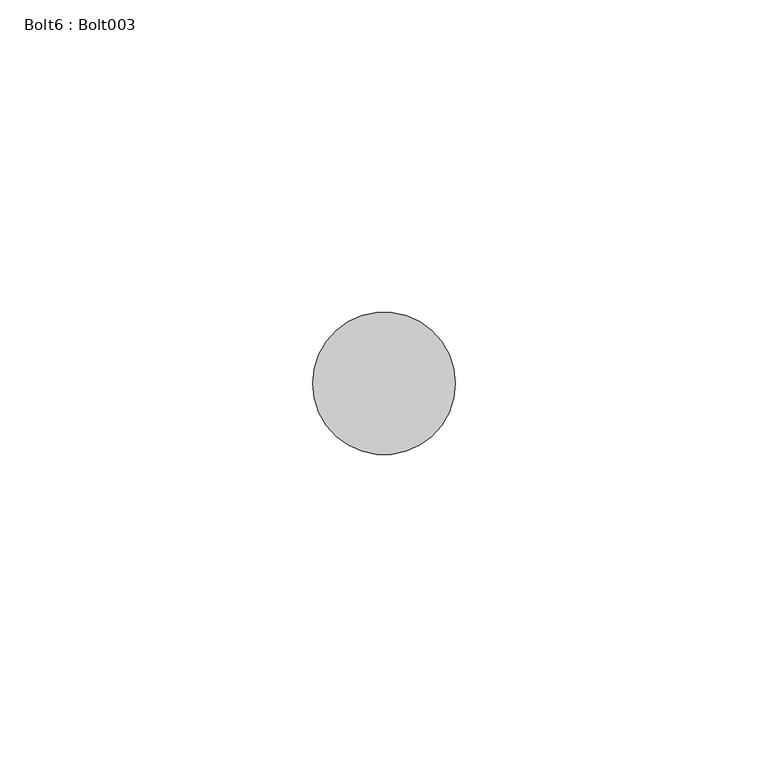
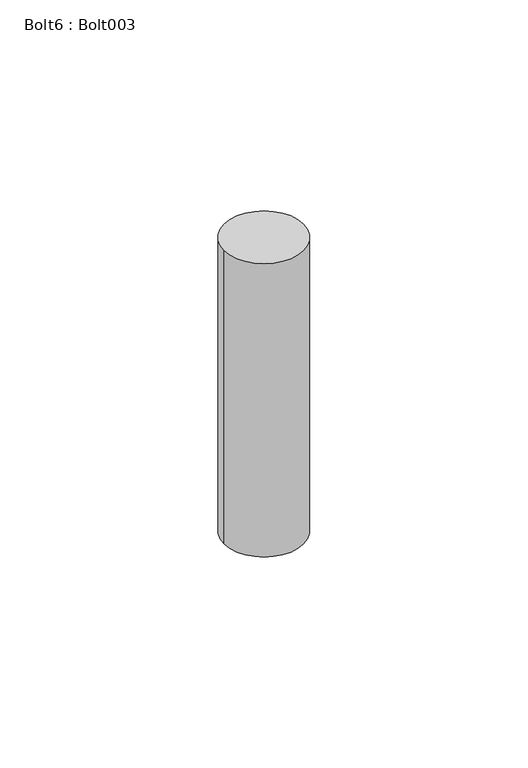
"""IFC4 building model written with IfcOpenShell, lengths in millimetres: proxy geometry, Bolt6 : Bolt003."""

from ifc_helpers import new_model, si_unit, point, frame, frame_2d, origin, place, context, project, spatial, circle_curve, trimmed, segment, composite_curve, outline, extrude, source, transform, mapped, element, save


def bolt6_bolt003_a672977d(model_context):
    return source(origin(), model_context, "Body", "SweptSolid", [
        extrude(outline(composite_curve([segment(trimmed(circle_curve(frame_2d((5172.3828124, 1896.5882072)), 11.4045168), [point((5160.9782956, 1896.5882072))], [point((5183.7873292, 1896.5882072))], False, "CARTESIAN"), True, "CONTINUOUS"), segment(trimmed(circle_curve(frame_2d((5172.3828124, 1896.5882072)), 11.4045168), [point((5183.7873292, 1896.5882072))], [point((5160.9782956, 1896.5882072))], False, "CARTESIAN"), True, "CONTINUOUS")], self_intersect=False)), frame((0.0, 0.0, 36645.5959962), z_axis=(0.0, 0.0, 1.0), x_axis=(1.0, 0.0, 0.0)), (0.0, 0.0, 1.0), 88.9),
    ])


if __name__ == "__main__":
    model = new_model("IFC4")
    model_context = context("Model", 3, world=origin())
    ifc_project = project(units=[si_unit("LENGTHUNIT", "METRE", prefix="MILLI")], contexts=[model_context])
    site = spatial("IfcSite", under=ifc_project)
    building = spatial("IfcBuilding", under=site)
    placement = place(None, origin())
    bolt6_bolt003_shape = bolt6_bolt003_a672977d(model_context)
    element("IfcBuildingElementProxy", 1, Name="Bolt6 : Bolt003", ObjectType="Bolt6 : Bolt003", at=placement, inside=building, context=model_context, shape_type="MappedRepresentation", body=[
        mapped(bolt6_bolt003_shape, transform((0.0, 0.0, 0.0), x_axis=(1.0, 0.0, 0.0), y_axis=(0.0, 1.0, 0.0), z_axis=(0.0, 0.0, 1.0))),
    ])
    save(model, "model.ifc")

# Revit data of these elements
# Type "Bolt6 : Bolt003"
#   NameOverride = "Bolt003"
# Element 1 (IfcBuildingElementProxy, "Bolt6 : Bolt003")
#   Materials on its faces: "TUBE STEEL STRINGER WELDED TO ANCHORED STEEL PLATE - SEE STRUCT DWGS"
# Materials
#   "TUBE STEEL STRINGER WELDED TO ANCHORED STEEL PLATE - SEE STRUCT DWGS": class "Unassigned", colour RGB 128 128 128, transparency 0, Cost = 0
